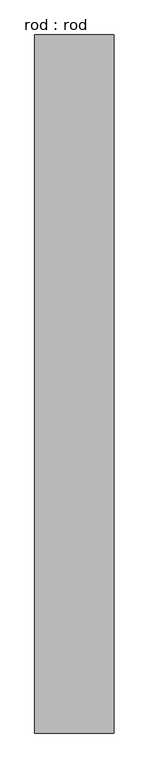
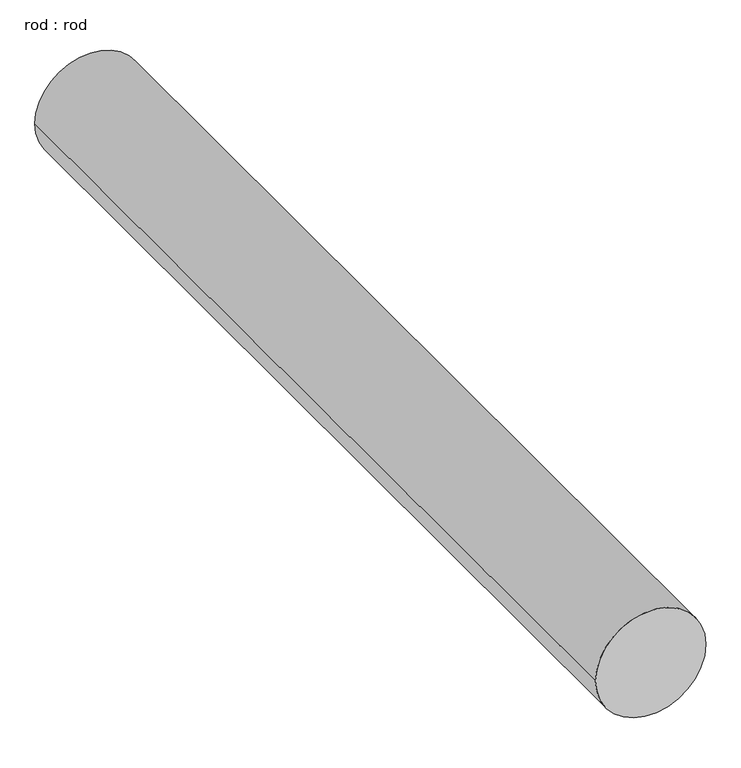
"""IFC4 building model written with IfcOpenShell, lengths in millimetres: proxy geometry, rod : rod."""

from ifc_helpers import new_model, si_unit, point, frame, frame_2d, origin, place, context, project, spatial, circle_curve, trimmed, segment, composite_curve, outline, extrude, source, transform, mapped, element, save


def rod_rod_4739a65c(model_context):
    return source(origin(), model_context, "Body", "SweptSolid", [
        extrude(outline(composite_curve([segment(trimmed(circle_curve(frame_2d((0.0108462, 0.0)), 200.0), [point((0.0108462, 200.0))], [point((0.0108462, -200.0))], False, "CARTESIAN"), True, "CONTINUOUS"), segment(trimmed(circle_curve(frame_2d((0.0108462, 0.0)), 200.0), [point((0.0108462, -200.0))], [point((0.0108462, 200.0))], False, "CARTESIAN"), True, "CONTINUOUS")], self_intersect=False)), frame((0.0, 2330.2286153, 0.0), z_axis=(0.0, 1.0, 0.0), x_axis=(0.0, 0.0, 1.0)), (0.0, 0.0, 1.0), 3525.0),
    ])


if __name__ == "__main__":
    model = new_model("IFC4")
    model_context = context("Model", 3, world=origin())
    ifc_project = project(units=[si_unit("LENGTHUNIT", "METRE", prefix="MILLI")], contexts=[model_context])
    site = spatial("IfcSite", under=ifc_project)
    building = spatial("IfcBuilding", under=site)
    placement = place(None, origin())
    rod_rod_shape = rod_rod_4739a65c(model_context)
    element("IfcBuildingElementProxy", 1, Name="rod : rod", ObjectType="rod : rod", at=placement, inside=building, context=model_context, shape_type="MappedRepresentation", body=[
        mapped(rod_rod_shape, transform((0.0, 0.0, 0.0), x_axis=(1.0, 0.0, 0.0), y_axis=(0.0, 1.0, 0.0), z_axis=(0.0, 0.0, 1.0))),
    ])
    save(model, "model.ifc")

# Revit data of these elements
# Type "rod : rod"
#   Default Elevation = 0
